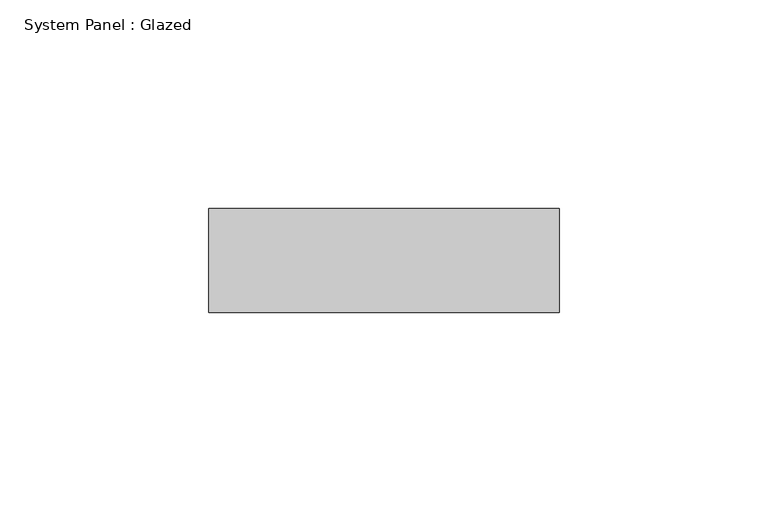
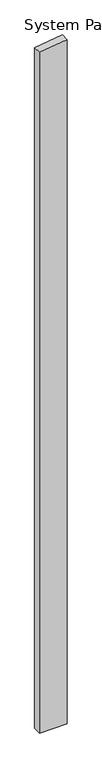
"""IFC4 building model written with IfcOpenShell, lengths in millimetres: plate geometry, System Panel : Glazed."""

from ifc_helpers import new_model, si_unit, frame, origin, place, context, project, spatial, polyline, outline, extrude, source, transform, mapped, element, save


def system_panel_glazed_658fc85f(model_context):
    return source(origin(), model_context, "Body", "SweptSolid", [
        extrude(outline(polyline([(0.0, -42.0223894), (0.0, 42.0223894), (300.0, 42.0223894), (2200.0, 42.0223894), (2188.0452602, -42.0223894), (0.0, -42.0223894)])), frame((0.0, 24.5, 0.0), z_axis=(0.0, 1.0, 0.0), x_axis=(0.0, 0.0, 1.0)), (0.0, 0.0, 1.0), 25.0),
    ])


if __name__ == "__main__":
    model = new_model("IFC4")
    model_context = context("Model", 3, world=origin())
    ifc_project = project(units=[si_unit("LENGTHUNIT", "METRE", prefix="MILLI")], contexts=[model_context])
    site = spatial("IfcSite", under=ifc_project)
    building = spatial("IfcBuilding", under=site)
    placement = place(None, origin())
    system_panel_glazed_shape = system_panel_glazed_658fc85f(model_context)
    element("IfcPlate", 1, ObjectType="System Panel : Glazed", at=placement, inside=building, context=model_context, shape_type="MappedRepresentation", body=[
        mapped(system_panel_glazed_shape, transform((0.0, 0.0, 0.0), x_axis=(1.0, 0.0, 0.0), y_axis=(0.0, 1.0, 0.0), z_axis=(0.0, 0.0, 1.0))),
    ])
    save(model, "model.ifc")

# Revit data of these elements
# Element 1 (IfcPlate, "System Panel : Glazed")
#   Materials on its faces: "Glass"
# Materials
#   "Glass": class "Glass", colour RGB 218 227 224, transparency 0.85, Description = "Soda Lime Glass", Cost = 0
